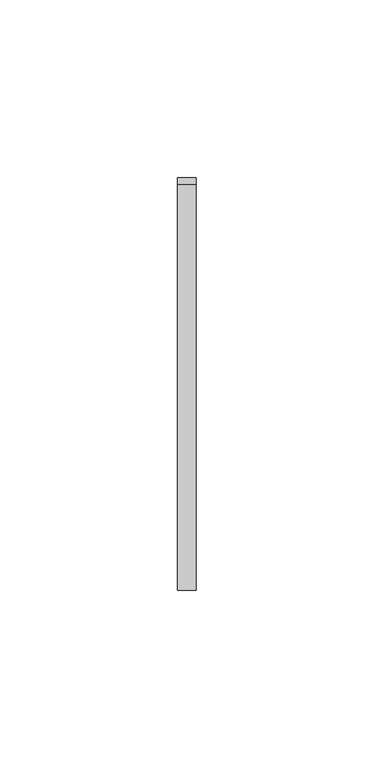
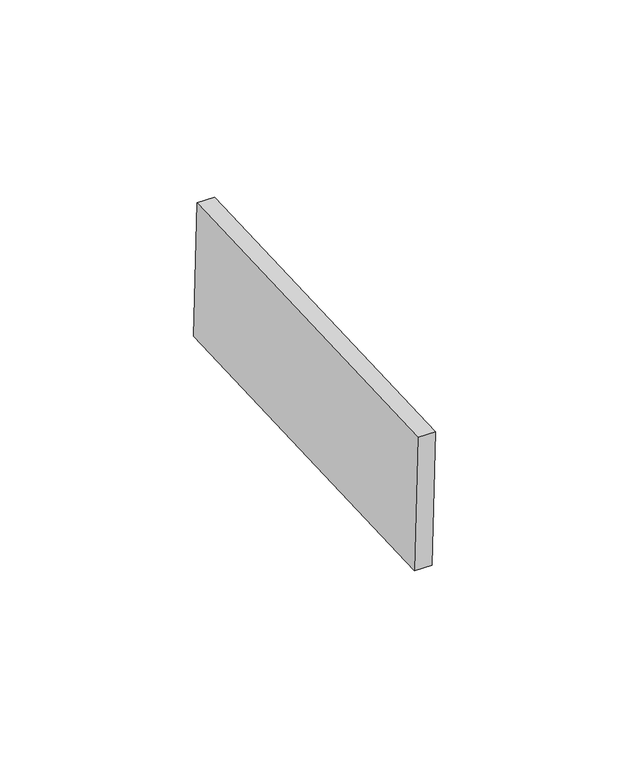
"""IFC4 building model written with IfcOpenShell, lengths in millimetres: proxy geometry, Inner panel:Inner panel:1:Inner panel:1 : Inner panel:Inner panel:300324:2:Inner panel:1:Inner panel:1 : Inner panel:Inner panel:300324:2 : Inner panel:Inner panel:1:Inner panel:1 : Inner panel:Inner panel:300324:300043:53 : Inner panel:Inner panel:1:Inner panel:1 : Inner panel:Inner panel:300324:2:Inner panel:1:Inner panel:1 : Inner panel:Inner panel:300324:2 : Inner panel:Inner panel:1:Inner panel:1 : Inner panel:Inner panel:300324:300043:308120."""

from ifc_helpers import new_model, si_unit, frame, origin, place, context, project, spatial, polyline, outline, extrude, source, transform, mapped, element, save


def generic_models_1038a89f(model_context):
    return source(origin(), model_context, "Body", "SweptSolid", [
        extrude(outline(polyline([(0.0, -114.2999999), (0.0, 0.0), (5.2138089, 0.0), (5.2138089, -114.2999999), (0.0, -114.2999999)])), frame((592717.395117, -566950.1308393, 8857.6957503), z_axis=(0.0, -0.04163054471215927, 0.9991330730923529), x_axis=(-1.0, 0.0, 0.0)), (0.0, 0.0, 1.0), 43.2233908),
    ])


if __name__ == "__main__":
    model = new_model("IFC4")
    model_context = context("Model", 3, world=origin())
    ifc_project = project(units=[si_unit("LENGTHUNIT", "METRE", prefix="MILLI")], contexts=[model_context])
    site = spatial("IfcSite", under=ifc_project)
    building = spatial("IfcBuilding", under=site)
    placement = place(None, origin())
    generic_models_shape = generic_models_1038a89f(model_context)
    element("IfcBuildingElementProxy", 1, Name="Inner panel:Inner panel:1:Inner panel:1 : Inner panel:Inner panel:300324:2:Inner panel:1:Inner panel:1 : Inner panel:Inner panel:300324:2 : Inner panel:Inner panel:1:Inner panel:1 : Inner panel:Inner panel:300324:300043:53 : Inner panel:Inner panel:1:Inner panel:1 : Inner panel:Inner panel:300324:2:Inner panel:1:Inner panel:1 : Inner panel:Inner panel:300324:2 : Inner panel:Inner panel:1:Inner panel:1 : Inner panel:Inner panel:300324:300043:308120", ObjectType="Inner panel:Inner panel:1:Inner panel:1 : Inner panel:Inner panel:300324:2:Inner panel:1:Inner panel:1 : Inner panel:Inner panel:300324:2 : Inner panel:Inner panel:1:Inner panel:1 : Inner panel:Inner panel:300324:300043:53 : Inner panel:Inner panel:1:Inner panel:1 : Inner panel:Inner panel:300324:2:Inner panel:1:Inner panel:1 : Inner panel:Inner panel:300324:2 : Inner panel:Inner panel:1:Inner panel:1 : Inner panel:Inner panel:300324:300043:308120", at=placement, inside=building, context=model_context, shape_type="MappedRepresentation", body=[
        mapped(generic_models_shape, transform((0.0, 0.0, 0.0), x_axis=(1.0, 0.0, 0.0), y_axis=(0.0, 1.0, 0.0), z_axis=(0.0, 0.0, 1.0))),
    ])
    save(model, "model.ifc")

# Revit data of these elements
# Type "Inner panel:Inner panel:1:Inner panel:1 : Inner panel:Inner panel:300324:2:Inner panel:1:Inner panel:1 : Inner panel:Inner panel:300324:2 : Inner panel:Inner panel:1:Inner panel:1 : Inner panel:Inner panel:300324:300043:53 : Inner panel:Inner panel:1:Inner panel:1 : Inner panel:Inner panel:300324:2:Inner panel:1:Inner panel:1 : Inner panel:Inner panel:300324:2 : Inner panel:Inner panel:1:Inner panel:1 : Inner panel:Inner panel:300324:300043:308120"
#   NameOverride = "Inner panel:Inner panel:1:Inner panel:1 : Inner panel:Inner panel:300324:2:Inner panel:1:Inner panel:1 : Inner panel:Inner panel:300324:2 : Inner panel:Inner panel:1:Inner panel:1 : Inner panel:Inner panel:300324:300043:308120"
#   ObjectTypeOverride = "Inner panel:1:Inner panel:1 : Inner panel:Inner panel:300324:2 : Inner panel:Inner panel:1:Inner panel:1 : Inner panel:Inner panel:300324:300043"
#   Reference = "Inner panel"
#   Tag = "308120"
# Element 1 (IfcBuildingElementProxy, "Inner panel:Inner panel:1:Inner panel:1 : Inner panel:Inner panel:300324:2:Inner panel:1:Inner panel:1 : Inner panel:Inner panel:300324:2 : Inner panel:Inner panel:1:Inner panel:1 : Inner panel:Inner panel:300324:300043:53 : Inner panel:Inner panel:1:Inner panel:1 : Inner panel:Inner panel:300324:2:Inner panel:1:Inner panel:1 : Inner panel:Inner panel:300324:2 : Inner panel:Inner panel:1:Inner panel:1 : Inner panel:Inner panel:300324:300043:308120")
#   Materials on its faces: "SLIDING CLIP"
# Materials
#   "SLIDING CLIP": class "Generic", colour RGB 120 120 120, transparency 0, Cost = 0
